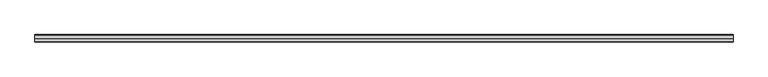
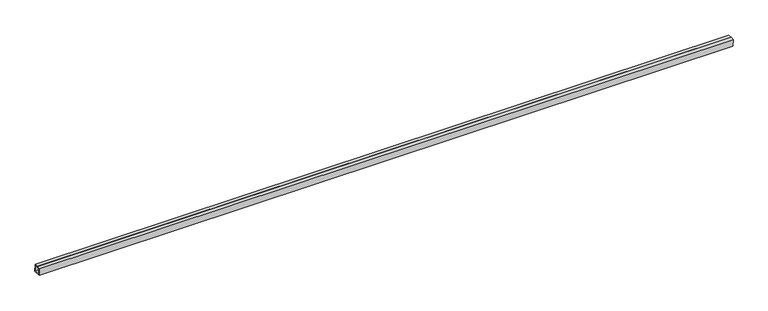
"""IFC4 building model written with IfcOpenShell, lengths in millimetres: proxy geometry, Inner panel:Inner panel:1:Inner panel:1 : Inner panel:Inner panel:300324:2:Inner panel:1:Inner panel:1 : Inner panel:Inner panel:300324:2 : Inner panel:Inner panel:1:Inner panel:1 : Inner panel:Inner panel:300324:300043:5 : Inner panel:Inner panel:1:Inner panel:1 : Inner panel:Inner panel:300324:2:Inner panel:1:Inner panel:1 : Inner panel:Inner panel:300324:2 : Inner panel:Inner panel:1:Inner panel:1 : Inner panel:Inner panel:300324:300043:308120."""

from ifc_helpers import new_model, si_unit, frame, origin, place, context, project, spatial, polyline, outline, extrude, source, transform, mapped, element, save


def generic_models_6b9c765e(model_context):
    return source(origin(), model_context, "Body", "SweptSolid", [
        extrude(outline(polyline([(-577873.8379638, 3996.8505773), (-577855.5975406, 3997.6105949), (-577854.0114169, 3959.5436248), (-577892.078387, 3957.9575011), (-577893.6645107, 3996.0244711), (-577875.4240875, 3996.7844888), (-577875.3249548, 3994.4053031), (-577891.1861923, 3993.7444182), (-577889.7983341, 3960.4358194), (-577856.4897352, 3961.8236777), (-577857.8775935, 3995.1322765), (-577873.7388311, 3994.4713916), (-577873.8379638, 3996.8505773)])), frame((593141.1867239, 0.0, 0.0), z_axis=(1.0, 0.0, 0.0), x_axis=(0.0, 1.0, 0.0)), (0.0, 0.0, 1.0), 3657.6),
    ])


if __name__ == "__main__":
    model = new_model("IFC4")
    model_context = context("Model", 3, world=origin())
    ifc_project = project(units=[si_unit("LENGTHUNIT", "METRE", prefix="MILLI")], contexts=[model_context])
    site = spatial("IfcSite", under=ifc_project)
    building = spatial("IfcBuilding", under=site)
    placement = place(None, origin())
    generic_models_shape = generic_models_6b9c765e(model_context)
    element("IfcBuildingElementProxy", 1, Name="Inner panel:Inner panel:1:Inner panel:1 : Inner panel:Inner panel:300324:2:Inner panel:1:Inner panel:1 : Inner panel:Inner panel:300324:2 : Inner panel:Inner panel:1:Inner panel:1 : Inner panel:Inner panel:300324:300043:5 : Inner panel:Inner panel:1:Inner panel:1 : Inner panel:Inner panel:300324:2:Inner panel:1:Inner panel:1 : Inner panel:Inner panel:300324:2 : Inner panel:Inner panel:1:Inner panel:1 : Inner panel:Inner panel:300324:300043:308120", ObjectType="Inner panel:Inner panel:1:Inner panel:1 : Inner panel:Inner panel:300324:2:Inner panel:1:Inner panel:1 : Inner panel:Inner panel:300324:2 : Inner panel:Inner panel:1:Inner panel:1 : Inner panel:Inner panel:300324:300043:5 : Inner panel:Inner panel:1:Inner panel:1 : Inner panel:Inner panel:300324:2:Inner panel:1:Inner panel:1 : Inner panel:Inner panel:300324:2 : Inner panel:Inner panel:1:Inner panel:1 : Inner panel:Inner panel:300324:300043:308120", at=placement, inside=building, context=model_context, shape_type="MappedRepresentation", body=[
        mapped(generic_models_shape, transform((0.0, 0.0, 0.0), x_axis=(1.0, 0.0, 0.0), y_axis=(0.0, 1.0, 0.0), z_axis=(0.0, 0.0, 1.0))),
    ])
    save(model, "model.ifc")

# Revit data of these elements
# Type "Inner panel:Inner panel:1:Inner panel:1 : Inner panel:Inner panel:300324:2:Inner panel:1:Inner panel:1 : Inner panel:Inner panel:300324:2 : Inner panel:Inner panel:1:Inner panel:1 : Inner panel:Inner panel:300324:300043:5 : Inner panel:Inner panel:1:Inner panel:1 : Inner panel:Inner panel:300324:2:Inner panel:1:Inner panel:1 : Inner panel:Inner panel:300324:2 : Inner panel:Inner panel:1:Inner panel:1 : Inner panel:Inner panel:300324:300043:308120"
#   NameOverride = "Inner panel:Inner panel:1:Inner panel:1 : Inner panel:Inner panel:300324:2:Inner panel:1:Inner panel:1 : Inner panel:Inner panel:300324:2 : Inner panel:Inner panel:1:Inner panel:1 : Inner panel:Inner panel:300324:300043:308120"
#   ObjectTypeOverride = "Inner panel:1:Inner panel:1 : Inner panel:Inner panel:300324:2 : Inner panel:Inner panel:1:Inner panel:1 : Inner panel:Inner panel:300324:300043"
#   Reference = "Inner panel"
#   Tag = "308120"
# Element 1 (IfcBuildingElementProxy, "Inner panel:Inner panel:1:Inner panel:1 : Inner panel:Inner panel:300324:2:Inner panel:1:Inner panel:1 : Inner panel:Inner panel:300324:2 : Inner panel:Inner panel:1:Inner panel:1 : Inner panel:Inner panel:300324:300043:5 : Inner panel:Inner panel:1:Inner panel:1 : Inner panel:Inner panel:300324:2:Inner panel:1:Inner panel:1 : Inner panel:Inner panel:300324:2 : Inner panel:Inner panel:1:Inner panel:1 : Inner panel:Inner panel:300324:300043:308120")
#   Materials on its faces: "1 1/2\" X 1 1/2\" SPLIT-SEAM SQUARE TUBING (~24\" CANTILEVER FROM C.L. OF GLULAM)"
# Materials
#   "1 1/2\" X 1 1/2\" SPLIT-SEAM SQUARE TUBING (~24\" CANTILEVER FROM C.L. OF GLULAM)": class "Unassigned", colour RGB 202 201 200, transparency 0, Cost = 0
